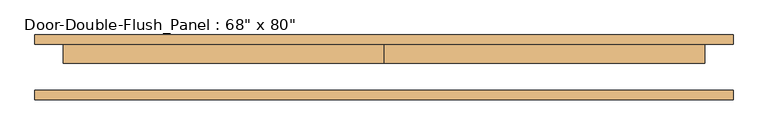
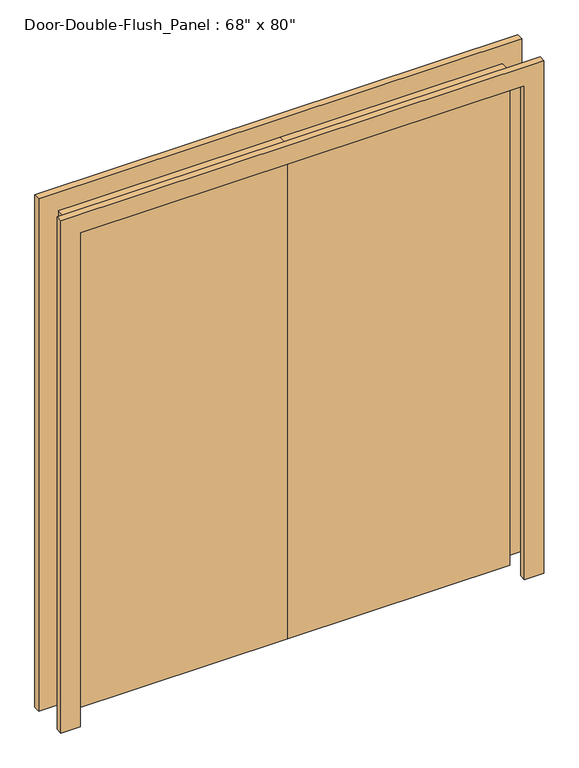
"""IFC4 building model written with IfcOpenShell, lengths in millimetres: door geometry."""

from ifc_helpers import new_model, si_unit, frame, origin, origin_with_axes, place, context, project, spatial, polyline, outline, extrude, source, transform, mapped, element, save


def door_7f6ceba9(model_context):
    return source(origin(), model_context, "Body", "SweptSolid", [
        extrude(outline(polyline([(2032.0, -863.6), (2032.0, 863.6), (0.0, 863.6), (0.0, 939.8), (2108.2, 939.8), (2108.2, -939.8), (0.0, -939.8), (0.0, -863.6), (2032.0, -863.6)])), frame((0.0, -87.3125, 0.0), z_axis=(0.0, 1.0, 0.0), x_axis=(0.0, 0.0, 1.0)), (0.0, 0.0, 1.0), 25.4),
        extrude(outline(polyline([(2032.0, -863.6), (2032.0, 863.6), (0.0, 863.6), (0.0, 939.8), (2108.2, 939.8), (2108.2, -939.8), (0.0, -939.8), (0.0, -863.6), (2032.0, -863.6)])), frame((0.0, 61.9125, 0.0), z_axis=(0.0, 1.0, 0.0), x_axis=(0.0, 0.0, 1.0)), (0.0, 0.0, 1.0), 25.4),
        extrude(outline(polyline([(0.0, 61.9125), (863.6, 61.9125), (863.6, 11.1125), (0.0, 11.1125), (0.0, 61.9125)])), origin_with_axes(), (0.0, 0.0, 1.0), 2032.0),
        extrude(outline(polyline([(-863.6, 61.9125), (0.0, 61.9125), (0.0, 11.1125), (-863.6, 11.1125), (-863.6, 61.9125)])), origin_with_axes(), (0.0, 0.0, 1.0), 2032.0),
    ])


if __name__ == "__main__":
    model = new_model("IFC4")
    model_context = context("Model", 3, world=origin())
    ifc_project = project(units=[si_unit("LENGTHUNIT", "METRE", prefix="MILLI")], contexts=[model_context])
    site = spatial("IfcSite", under=ifc_project)
    building = spatial("IfcBuilding", under=site)
    placement = place(None, origin())
    door_shape = door_7f6ceba9(model_context)
    element("IfcDoor", 1, ObjectType="Door-Double-Flush_Panel : 68\" x 80\"", at=placement, inside=building, context=model_context, shape_type="MappedRepresentation", body=[
        mapped(door_shape, transform((0.0, 0.0, 0.0), x_axis=(1.0, 0.0, 0.0), y_axis=(0.0, 1.0, 0.0), z_axis=(0.0, 0.0, 1.0))),
    ])
    save(model, "model.ifc")

# Revit data of these elements
# Type "Door-Double-Flush_Panel : 68\" x 80\""
#   Type Mark = "8"
#   Construction Type Id = "DOOR"
#   Assembly Code = "C1020"
#   Analytic Construction = "Wooden"
#   Thickness = 0' - 2"
#   Thermal Resistance (R) = 0.455703 (m²·K)/W
#   Swing Angle [instance default] = 90.00°
#   Panel Width = 2' - 10"
#   Heat Transfer Coefficient (U) = 2.19465 W/(m²·K)
#   Height = 6' - 8"
#   Trim Projection Ext = 0' - 1"
#   Trim Projection Int = 0' - 1"
#   Trim Width = 0' - 3"
#   Width = 5' - 8"
#   Panel Material = Wood - Birch - Solid Stained Light Low Gloss
#   Trim Material = Paint - Sienna
#   Visual Light Transmittance = 0
#   Solar Heat Gain Coefficient = 0
#   Function = (empty or 0)
#   Wall Closure = (empty or 0)
# Element 1 (IfcDoor, "Door-Double-Flush_Panel : 68\" x 80\"")
#   Materials on its faces: "Paint - Sienna", "Wood - Birch - Solid Stained Light Low Gloss"
# Materials
#   "Wood - Birch - Solid Stained Light Low Gloss": class "Wood", colour RGB 210 159 95, transparency 0, Cost = 0
#   "Paint - Sienna": class "Miscellaneous", colour RGB 118 70 51, transparency 0, Cost = 0
